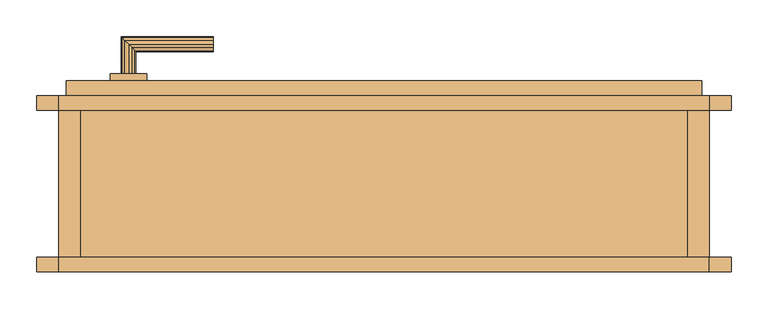
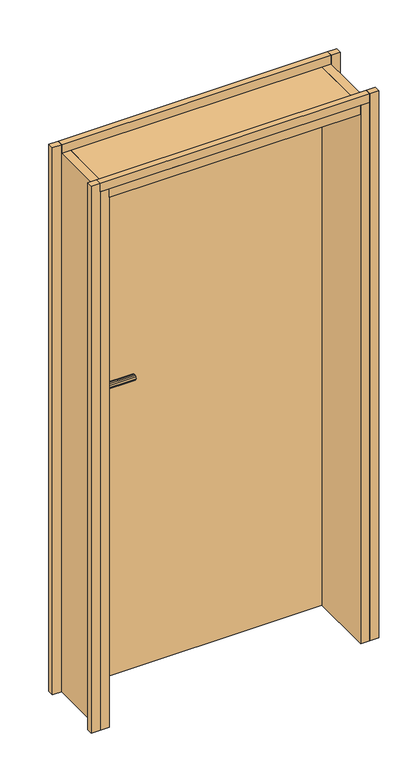
"""IFC4 building model written with IfcOpenShell, lengths in millimetres: door geometry, Tür."""

from ifc_helpers import new_model, si_unit, frame, origin, place, context, project, spatial, polyline, outline, extrude, faceted_brep, source, transform, mapped, element, save


def door_1d95d05b(model_context):
    return source(origin(), model_context, "Body", "SolidModel", [
        extrude(outline(polyline([(885.0, 200.0), (0.0, 200.0), (0.0, 220.0), (885.0, 220.0), (885.0, 200.0)])), frame((0.0, 0.0, 2010.0), z_axis=(0.0, 0.0, 1.0), x_axis=(1.0, 0.0, 0.0)), (0.0, 0.0, 1.0), 30.0),
        faceted_brep([(100.0, 250.0, 1198.660254), (95.0, 250.0, 1200.0), (90.0, 250.0, 1198.660254), (86.339746, 250.0, 1195.0), (85.0, 250.0, 1190.0), (86.339746, 250.0, 1185.0), (90.0, 250.0, 1181.339746), (95.0, 250.0, 1180.0), (100.0, 250.0, 1181.339746), (103.660254, 250.0, 1185.0), (105.0, 250.0, 1190.0), (103.660254, 250.0, 1195.0), (95.0, 290.0, 1200.0), (90.0, 295.0, 1198.660254), (86.339746, 298.660254, 1195.0), (85.0, 300.0, 1190.0), (86.339746, 298.660254, 1185.0), (90.0, 295.0, 1181.339746), (95.0, 290.0, 1180.0), (100.0, 285.0, 1181.339746), (103.660254, 281.339746, 1185.0), (105.0, 280.0, 1190.0), (103.660254, 281.339746, 1195.0), (100.0, 285.0, 1198.660254), (210.0, 295.0, 1198.660254), (210.0, 290.0, 1200.0), (210.0, 285.0, 1198.660254), (210.0, 281.339746, 1195.0), (210.0, 280.0, 1190.0), (210.0, 281.339746, 1185.0), (210.0, 285.0, 1181.339746), (210.0, 290.0, 1180.0), (210.0, 295.0, 1181.339746), (210.0, 298.660254, 1185.0), (210.0, 300.0, 1190.0), (210.0, 298.660254, 1195.0)], [[[0, 1, 2, 3, 4, 5, 6, 7, 8, 9, 10, 11]], [[2, 1, 12, 13]], [[3, 2, 13, 14]], [[4, 3, 14, 15]], [[5, 4, 15, 16]], [[6, 5, 16, 17]], [[7, 6, 17, 18]], [[8, 7, 18, 19]], [[9, 8, 19, 20]], [[10, 9, 20, 21]], [[11, 10, 21, 22]], [[0, 11, 22, 23]], [[1, 0, 23, 12]], [[24, 25, 26, 27, 28, 29, 30, 31, 32, 33, 34, 35]], [[13, 12, 25, 24]], [[14, 13, 24, 35]], [[15, 14, 35, 34]], [[16, 15, 34, 33]], [[17, 16, 33, 32]], [[18, 17, 32, 31]], [[19, 18, 31, 30]], [[20, 19, 30, 29]], [[21, 20, 29, 28]], [[22, 21, 28, 27]], [[23, 22, 27, 26]], [[12, 23, 26, 25]]]),
        extrude(outline(polyline([(915.0, 0.0), (915.0, -20.0), (885.0, -20.0), (885.0, 0.0), (915.0, 0.0)])), frame((0.0, 0.0, 140.0), z_axis=(0.0, 0.0, 1.0), x_axis=(1.0, 0.0, 0.0)), (0.0, 0.0, 1.0), 1900.0),
        extrude(outline(polyline([(70.0, 190.0), (70.0, 200.0), (120.0, 200.0), (120.0, 190.0), (70.0, 190.0)])), frame((0.0, 0.0, 1050.0), z_axis=(0.0, 0.0, 1.0), x_axis=(1.0, 0.0, 0.0)), (0.0, 0.0, 1.0), 215.0),
        extrude(outline(polyline([(885.0, -20.0), (0.0, -20.0), (0.0, 0.0), (885.0, 0.0), (885.0, -20.0)])), frame((0.0, 0.0, 2010.0), z_axis=(0.0, 0.0, 1.0), x_axis=(1.0, 0.0, 0.0)), (0.0, 0.0, 1.0), 30.0),
        extrude(outline(polyline([(875.0, 200.0), (10.0, 200.0), (10.0, 240.0), (875.0, 240.0), (875.0, 200.0)])), frame((0.0, 0.0, 140.0), z_axis=(0.0, 0.0, 1.0), x_axis=(1.0, 0.0, 0.0)), (0.0, 0.0, 1.0), 1860.0),
        extrude(outline(polyline([(0.0, -20.0), (-30.0, -20.0), (-30.0, 0.0), (0.0, 0.0), (0.0, -20.0)])), frame((0.0, 0.0, 140.0), z_axis=(0.0, 0.0, 1.0), x_axis=(1.0, 0.0, 0.0)), (0.0, 0.0, 1.0), 1900.0),
        extrude(outline(polyline([(915.0, 220.0), (915.0, 200.0), (885.0, 200.0), (885.0, 220.0), (915.0, 220.0)])), frame((0.0, 0.0, 140.0), z_axis=(0.0, 0.0, 1.0), x_axis=(1.0, 0.0, 0.0)), (0.0, 0.0, 1.0), 1900.0),
        extrude(outline(polyline([(855.0, -20.0), (30.0, -20.0), (30.0, 220.0), (855.0, 220.0), (855.0, -20.0)])), frame((0.0, 0.0, 1980.0), z_axis=(0.0, 0.0, 1.0), x_axis=(1.0, 0.0, 0.0)), (0.0, 0.0, 1.0), 30.0),
        extrude(outline(polyline([(120.0, 240.0), (70.0, 240.0), (70.0, 250.0), (120.0, 250.0), (120.0, 240.0)])), frame((0.0, 0.0, 1050.0), z_axis=(0.0, 0.0, 1.0), x_axis=(1.0, 0.0, 0.0)), (0.0, 0.0, 1.0), 215.0),
        extrude(outline(polyline([(30.0, -20.0), (0.0, -20.0), (0.0, 220.0), (30.0, 220.0), (30.0, -20.0)])), frame((0.0, 0.0, 140.0), z_axis=(0.0, 0.0, 1.0), x_axis=(1.0, 0.0, 0.0)), (0.0, 0.0, 1.0), 1870.0),
        extrude(outline(polyline([(885.0, -20.0), (855.0, -20.0), (855.0, 220.0), (885.0, 220.0), (885.0, -20.0)])), frame((0.0, 0.0, 140.0), z_axis=(0.0, 0.0, 1.0), x_axis=(1.0, 0.0, 0.0)), (0.0, 0.0, 1.0), 1870.0),
        extrude(outline(polyline([(0.0, 200.0), (-30.0, 200.0), (-30.0, 220.0), (0.0, 220.0), (0.0, 200.0)])), frame((0.0, 0.0, 140.0), z_axis=(0.0, 0.0, 1.0), x_axis=(1.0, 0.0, 0.0)), (0.0, 0.0, 1.0), 1900.0),
        faceted_brep([(90.0, 190.0, 1198.660254), (95.0, 190.0, 1200.0), (100.0, 190.0, 1198.660254), (103.660254, 190.0, 1195.0), (105.0, 190.0, 1190.0), (103.660254, 190.0, 1185.0), (100.0, 190.0, 1181.339746), (95.0, 190.0, 1180.0), (90.0, 190.0, 1181.339746), (86.339746, 190.0, 1185.0), (85.0, 190.0, 1190.0), (86.339746, 190.0, 1195.0), (95.0, 150.0, 1200.0), (90.0, 145.0, 1198.660254), (86.339746, 141.339746, 1195.0), (85.0, 140.0, 1190.0), (86.339746, 141.339746, 1185.0), (90.0, 145.0, 1181.339746), (95.0, 150.0, 1180.0), (100.0, 155.0, 1181.339746), (103.660254, 158.660254, 1185.0), (105.0, 160.0, 1190.0), (103.660254, 158.660254, 1195.0), (100.0, 155.0, 1198.660254), (210.0, 155.0, 1198.660254), (210.0, 150.0, 1200.0), (210.0, 145.0, 1198.660254), (210.0, 141.339746, 1195.0), (210.0, 140.0, 1190.0), (210.0, 141.339746, 1185.0), (210.0, 145.0, 1181.339746), (210.0, 150.0, 1180.0), (210.0, 155.0, 1181.339746), (210.0, 158.660254, 1185.0), (210.0, 160.0, 1190.0), (210.0, 158.660254, 1195.0)], [[[0, 1, 2, 3, 4, 5, 6, 7, 8, 9, 10, 11]], [[12, 1, 0, 13]], [[13, 0, 11, 14]], [[14, 11, 10, 15]], [[15, 10, 9, 16]], [[16, 9, 8, 17]], [[17, 8, 7, 18]], [[18, 7, 6, 19]], [[19, 6, 5, 20]], [[20, 5, 4, 21]], [[21, 4, 3, 22]], [[22, 3, 2, 23]], [[23, 2, 1, 12]], [[24, 25, 26, 27, 28, 29, 30, 31, 32, 33, 34, 35]], [[25, 12, 13, 26]], [[26, 13, 14, 27]], [[27, 14, 15, 28]], [[28, 15, 16, 29]], [[29, 16, 17, 30]], [[30, 17, 18, 31]], [[31, 18, 19, 32]], [[32, 19, 20, 33]], [[33, 20, 21, 34]], [[34, 21, 22, 35]], [[35, 22, 23, 24]], [[24, 23, 12, 25]]]),
    ])


if __name__ == "__main__":
    model = new_model("IFC4")
    model_context = context("Model", 3, world=origin())
    ifc_project = project(units=[si_unit("LENGTHUNIT", "METRE", prefix="MILLI")], contexts=[model_context])
    site = spatial("IfcSite", under=ifc_project)
    building = spatial("IfcBuilding", under=site)
    placement = place(None, origin())
    door_shape = door_1d95d05b(model_context)
    element("IfcDoor", 1, ObjectType="Tür", at=placement, inside=building, context=model_context, shape_type="MappedRepresentation", body=[
        mapped(door_shape, transform((0.0, 0.0, 0.0), x_axis=(1.0, 0.0, 0.0), y_axis=(0.0, 1.0, 0.0), z_axis=(0.0, 0.0, 1.0))),
    ])
    save(model, "model.ifc")

# Revit data of these elements
# Type "Tür"
#   Type Mark = "47"
# Element 1 (IfcDoor, "Tür")
#   Materials on its faces: "tuer_beschlag", "tuer_holzzarge"
# Materials
#   "tuer_beschlag": class "Unassigned", colour RGB 128 128 128, transparency 0
#   "tuer_holzzarge": class "Unassigned", colour RGB 255 255 255, transparency 0
